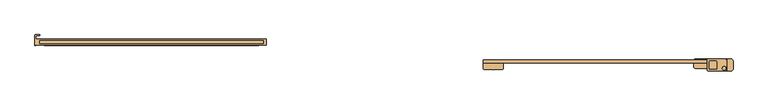
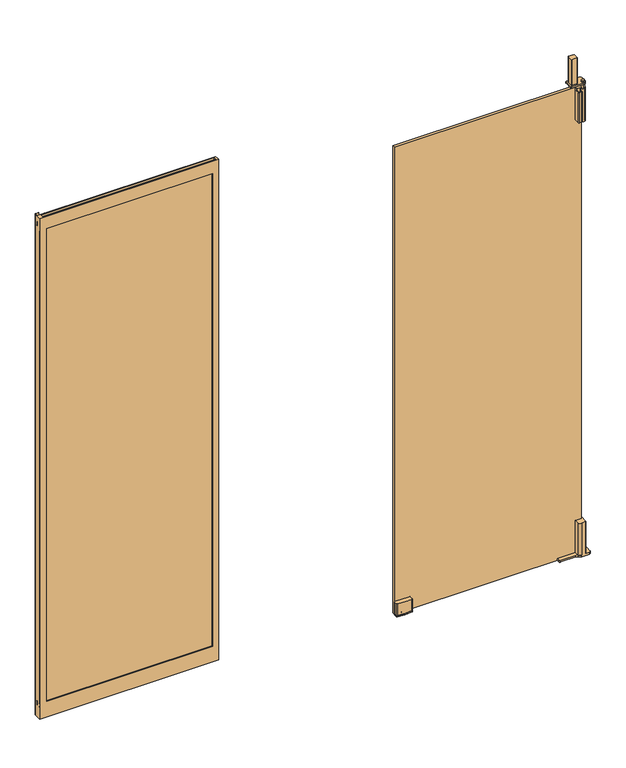
# IFC4 building model written with IfcOpenShell, lengths in millimetres: door geometry, Otomatik Kapı-Çift Kanat : Otomatik Kapı - Çift Kanat - 150-220.
# Revit data of these elements (continued)
# Type "Otomatik Kapı-Çift Kanat : Otomatik Kapı - Çift Kanat - 150-220" (continued)
#   Bottom Rail Note 2 [instance default] = "For the Drained continuous guide rail There must be flexible tubes on site to take out water (Slope < 1.5 %). The flexible tube connection is thread ½, and a EPDM foil or liquid synthetic material outside and a Air- and vapor-tight foil inside (on site)"
#   Bottom Rail Note [instance default] = "For drained and heated rails a cable from the header to the bottom rail in a M25 pipe is needed"
#   BIMobject category = "Sliding"
#   Assembly Code = "B2030100"
#   Analytic Construction = "<None>"
#   Standard Profile [instance default] = 0.00 cm
#   Rough Width = 300.00 cm
#   Rough Height [instance default] = 234.00 cm
#   Post Width = 150.84 cm
#   Pocket screen width R = 78.82 cm
#   Pocket screen width L = 78.82 cm
#   Pocket screen height [instance default] = 222.50 cm
#   Openning distance [instance default] = 3.09 cm
#   Opening Width LB = 150.00 cm
#   Opening Width Control = 150.00 cm
#   Opening Height LH = 220.00 cm
#   Moving leaf width = 75.42 cm
#   Moving leaf height [instance default] = 224.10 cm
#   Inset [instance default] = 0.00 cm
#   Header width = 299.50 cm
#   Header offset right CR = 0.00 cm
#   Header offset left CL = 0.00 cm
#   Header height [instance default] = 14.00 cm
#   Header depth [instance default] = 22.50 cm
#   Header Right Control = 0.00 cm
#   Header Left Control = 0.00 cm
#   Gap above header control [instance default] = 0.00 cm
#   Gap above header OH = 0.00 cm
#   Gap = 0.00 cm
#   Height = 220.00 cm
#   Width = 300.00 cm
#   Fixed leaf height [instance default] = 223.20 cm
#   Fixed leaf R width = 75.42 cm
#   Fixed leaf L width = 75.42 cm
#   CR max = 300.00 cm
#   CL max = 300.00 cm
#   Standard [instance default] = no
#   Side plate [instance default] = no
#   Side cap [instance default] = yes
#   Rail 4 [instance default] = no
#   Rail 3 [instance default] = no
#   Rail 2 [instance default] = no
#   Rail 1 [instance default] = no
#   Pocket screen [instance default] = yes
#   Open [instance default] = no
#   Heated [instance default] = no
#   Fixed point [instance default] = yes
#   Edition number = 1
#   Dimensions overconstraint = no
#   Connector [instance default] = no
#   Closing Profile [instance default] = yes
#   Mounting Option [instance default] = element 451667
#   Mounting G = element 451673
#   Mounting F = element 451672
#   Mounting E = element 451671
#   Mounting D = element 451670
#   Mounting C = element 451669
#   Mounting B = element 451668
#   Mounting A = element 451667
#   Header Option [instance default] = element 451680
#   Header 2 = element 451680
#   Header 1 = element 451679
#   Guide 5 = element 451678
#   Guide 4 = element 451674
#   Guide 3 = element 451677
#   Guide 2 = element 451676
#   Guide 1 = element 451675
#   Frame material = Finish_Gilgen_Aluminium
#   Bottom Guide Rail [instance default] = element 451674
#   Function = (empty or 0)
#   Wall Closure = (empty or 0)
# Element 1 (IfcDoor, "Otomatik Kapı-Çift Kanat : Otomatik Kapı - Çift Kanat - 150-220")
#   Materials on its faces: "Finish_Gilgen_Aluminium", "Glass", "Rubber, Natural", "Plastic, Opaque Black"
# Materials
#   "Finish_Gilgen_Aluminium": class "Metal", colour RGB 120 120 120, transparency 0, Description = "Aluminium", Cost = 0
#   "Glass": class "Glass", colour RGB 0 128 192, transparency 0.9, Description = "Soda Lime Glass", Cost = 0
#   "Rubber, Natural": class "Plastic", colour RGB 120 120 120, transparency 0, Description = "Natural rubber", Cost = 0
#   "Plastic, Opaque Black": class "Plastic", colour RGB 120 120 120, transparency 0, Description = "Plastic, generic, opaque black", Cost = 0
